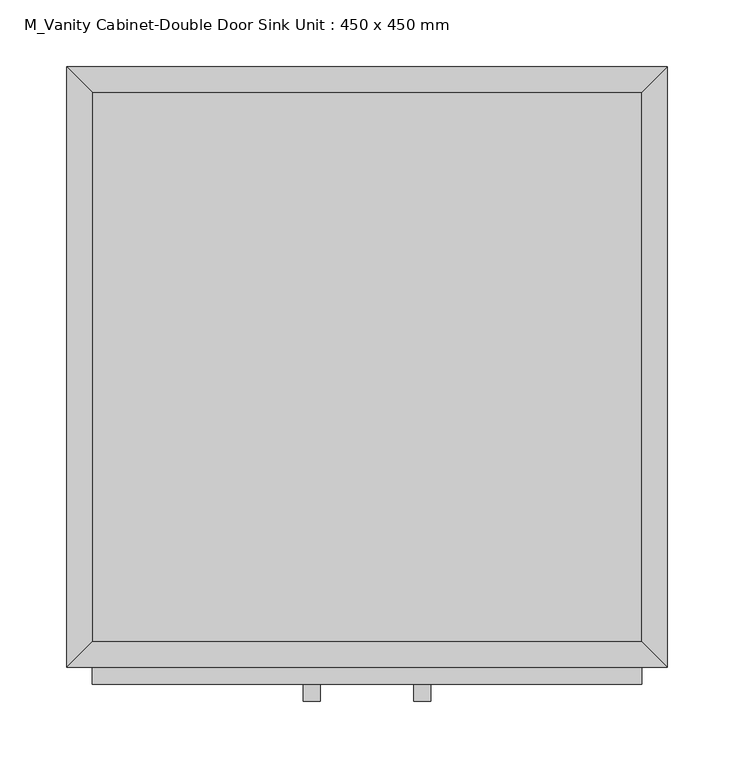
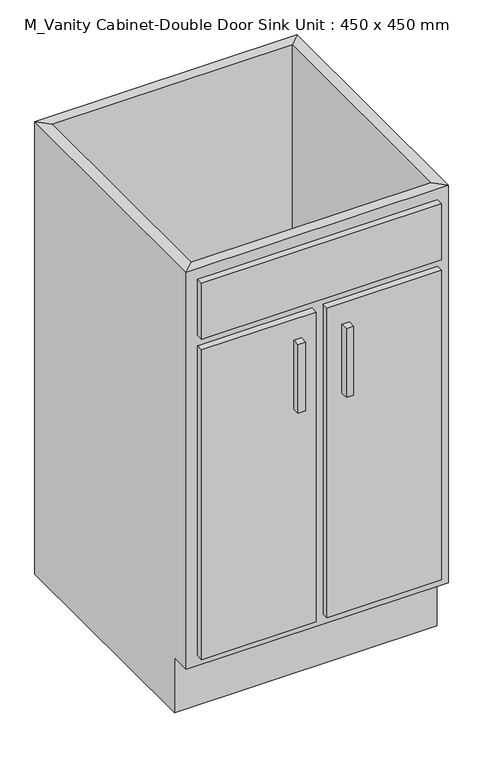
"""IFC4 building model written with IfcOpenShell, lengths in millimetres: furniture geometry, M_Vanity Cabinet-Double Door Sink Unit : 450 x 450 mm."""

from ifc_helpers import new_model, si_unit, frame, origin, place, context, project, spatial, polyline, outline, extrude, faceted_brep, source, transform, mapped, element, save


def m_vanity_cabinet_double_door_sink_unit_450_x_450_mm_cc3f0d44(model_context):
    return source(origin(), model_context, "Body", "SolidModel", [
        faceted_brep([(224.6877049, -430.95, 820.0), (224.6877049, -430.95, 100.0), (-187.2122951, -430.95, 100.0), (-187.2122951, -430.95, 820.0), (-206.2622951, -450.0, 820.0), (243.7377049, -450.0, 820.0), (-206.2622951, -450.0, 100.0), (243.7377049, -450.0, 100.0), (-187.2122951, -415.0, 100.0), (-187.2122951, -19.05, 100.0), (-187.2122951, -19.05, 820.0), (-206.2622951, 0.0, 820.0), (-206.2622951, 0.0, 0.0), (-206.2622951, -415.0, 0.0), (-206.2622951, -415.0, 100.0), (224.6877049, -19.05, 100.0), (224.6877049, -19.05, 820.0), (243.7377049, 0.0, 820.0), (243.7377049, 0.0, 0.0), (224.6877049, -415.0, 100.0), (243.7377049, -415.0, 100.0), (243.7377049, -415.0, 0.0)], [[[0, 1, 2, 3]], [[0, 3, 4, 5]], [[5, 4, 6, 7]], [[2, 1, 7, 6]], [[3, 2, 8, 9, 10]], [[4, 3, 10, 11]], [[6, 4, 11, 12, 13, 14]], [[2, 6, 14, 8]], [[10, 9, 15, 16]], [[11, 10, 16, 17]], [[12, 11, 17, 18]], [[1, 0, 16, 15, 19]], [[0, 5, 17, 16]], [[5, 7, 20, 21, 18, 17]], [[7, 1, 19, 20]], [[8, 19, 15, 9]], [[18, 21, 13, 12]], [[13, 21, 20, 19, 8, 14]]]),
        extrude(outline(polyline([(-16.1872951, -475.4), (-28.8872951, -475.4), (-28.8872951, -462.7), (-16.1872951, -462.7), (-16.1872951, -475.4)])), frame((0.0, 0.0, 517.469895), z_axis=(0.0, 0.0, 1.0), x_axis=(1.0, 0.0, 0.0)), (0.0, 0.0, 1.0), 124.730105),
        extrude(outline(polyline([(66.3627049, -475.4), (53.6627049, -475.4), (53.6627049, -462.7), (66.3627049, -462.7), (66.3627049, -475.4)])), frame((0.0, 0.0, 517.469895), z_axis=(0.0, 0.0, 1.0), x_axis=(1.0, 0.0, 0.0)), (0.0, 0.0, 1.0), 124.730105),
        extrude(outline(polyline([(9.2127049, -462.7), (-187.2122951, -462.7), (-187.2122951, -450.0), (9.2127049, -450.0), (9.2127049, -462.7)])), frame((0.0, 0.0, 119.05), z_axis=(0.0, 0.0, 1.0), x_axis=(1.0, 0.0, 0.0)), (0.0, 0.0, 1.0), 561.25),
        extrude(outline(polyline([(224.6877049, -462.7), (28.2627049, -462.7), (28.2627049, -450.0), (224.6877049, -450.0), (224.6877049, -462.7)])), frame((0.0, 0.0, 119.05), z_axis=(0.0, 0.0, 1.0), x_axis=(1.0, 0.0, 0.0)), (0.0, 0.0, 1.0), 561.25),
        extrude(outline(polyline([(224.6877049, -462.7), (-187.2122951, -462.7), (-187.2122951, -450.0), (224.6877049, -450.0), (224.6877049, -462.7)])), frame((0.0, 0.0, 699.35), z_axis=(0.0, 0.0, 1.0), x_axis=(1.0, 0.0, 0.0)), (0.0, 0.0, 1.0), 101.6),
        extrude(outline(polyline([(224.6877049, -19.05), (224.6877049, -430.95), (-187.2122951, -430.95), (-187.2122951, -19.05), (224.6877049, -19.05)])), frame((0.0, 0.0, 100.0), z_axis=(0.0, 0.0, 1.0), x_axis=(1.0, 0.0, 0.0)), (0.0, 0.0, 1.0), 19.05),
    ])


if __name__ == "__main__":
    model = new_model("IFC4")
    model_context = context("Model", 3, world=origin())
    ifc_project = project(units=[si_unit("LENGTHUNIT", "METRE", prefix="MILLI")], contexts=[model_context])
    site = spatial("IfcSite", under=ifc_project)
    building = spatial("IfcBuilding", under=site)
    placement = place(None, origin())
    m_vanity_cabinet_double_door_sink_unit_450_x_450_mm_shape = m_vanity_cabinet_double_door_sink_unit_450_x_450_mm_cc3f0d44(model_context)
    element("IfcFurniture", 1, ObjectType="M_Vanity Cabinet-Double Door Sink Unit : 450 x 450 mm", at=placement, inside=building, context=model_context, shape_type="MappedRepresentation", body=[
        mapped(m_vanity_cabinet_double_door_sink_unit_450_x_450_mm_shape, transform((0.0, 0.0, 0.0), x_axis=(1.0, 0.0, 0.0), y_axis=(0.0, 1.0, 0.0), z_axis=(0.0, 0.0, 1.0))),
    ])
    save(model, "model.ifc")

# Revit data of these elements
# Type "M_Vanity Cabinet-Double Door Sink Unit : 450 x 450 mm"
#   Manufacturer = "Manufacturer"
#   Finish = "Finish"
#   Construction Type = "Construction Type"
#   AccessibilityPerformance = "AccessibilityPerformance"
#   CodePerformance = "CodePerformance"
#   Area = "Area"
#   Color = "Color"
#   Constituents = "Constituents"
#   Features = "Features"
#   Finish = "Finish"
#   Grade = "Grade"
#   Material = "Material"
#   ModelReference = "ModelReference"
#   NominalHeight = "NominalHeight"
#   NominalLength = "NominalLength"
#   NominalWidth = "NominalWidth"
#   ProductionYear = "ProductionYear"
#   Reference = "Reference"
#   Shape = "Shape"
#   Size = "Size"
#   SustainabilityPerformance = "SustainabilityPerformance"
#   WarrantyDescription = "WarrantyDescription"
#   WarrantyDurationLabor = "WarrantyDurationLabor"
#   WarrantyDurationParts = "WarrantyDurationParts"
#   WarrantyGuarantorLabor = "WarrantyGuarantorLabor"
#   WarrantyGuarantorParts = "WarrantyGuarantorParts"
#   ExpectedLife = "ExpectedLife"
#   ReplacementCost = "ReplacementCost"
#   AssetAccountingType = "FIXED"
#   ModelLabel = "ModelLabel"
#   Depth = 0.450 m
#   Height = 0.820 m
#   Plinth Depth = 0.035 m
#   Plinth Height = 0.100 m
#   Width = 0.450 m
#   Cabinet Material = none
#   Door/Drawer Material = none
#   Handle Material = Cabinets - Handles
# Element 1 (IfcFurniture, "M_Vanity Cabinet-Double Door Sink Unit : 450 x 450 mm")
#   Materials on its faces: "Cabinets", "Cabinets - Handles"
# Materials
#   "Cabinets - Handles": class "Metal", colour RGB 57 57 57, transparency 0
#   "Cabinets": class "Miscellaneous", colour RGB 249 249 249, transparency 0
